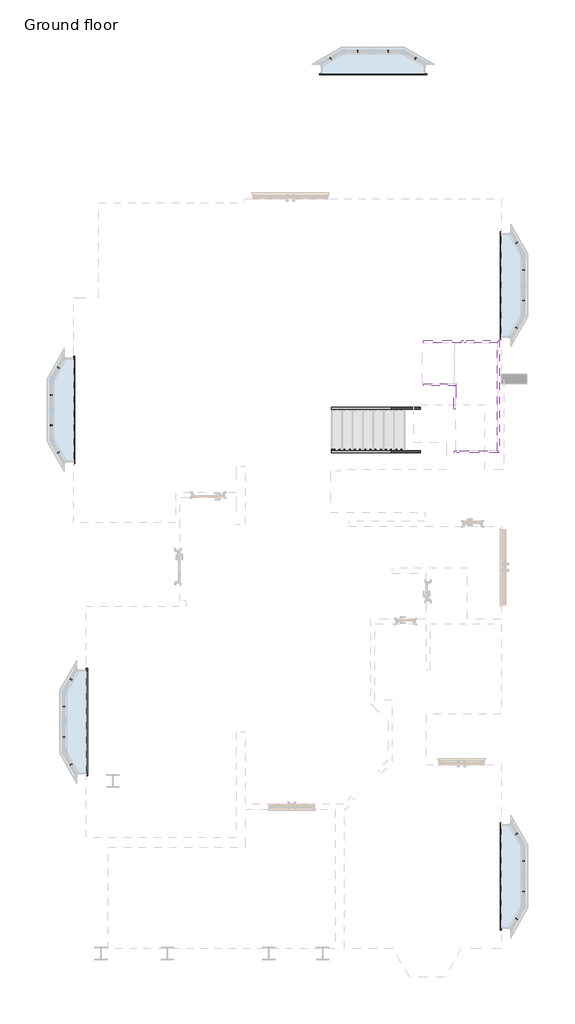
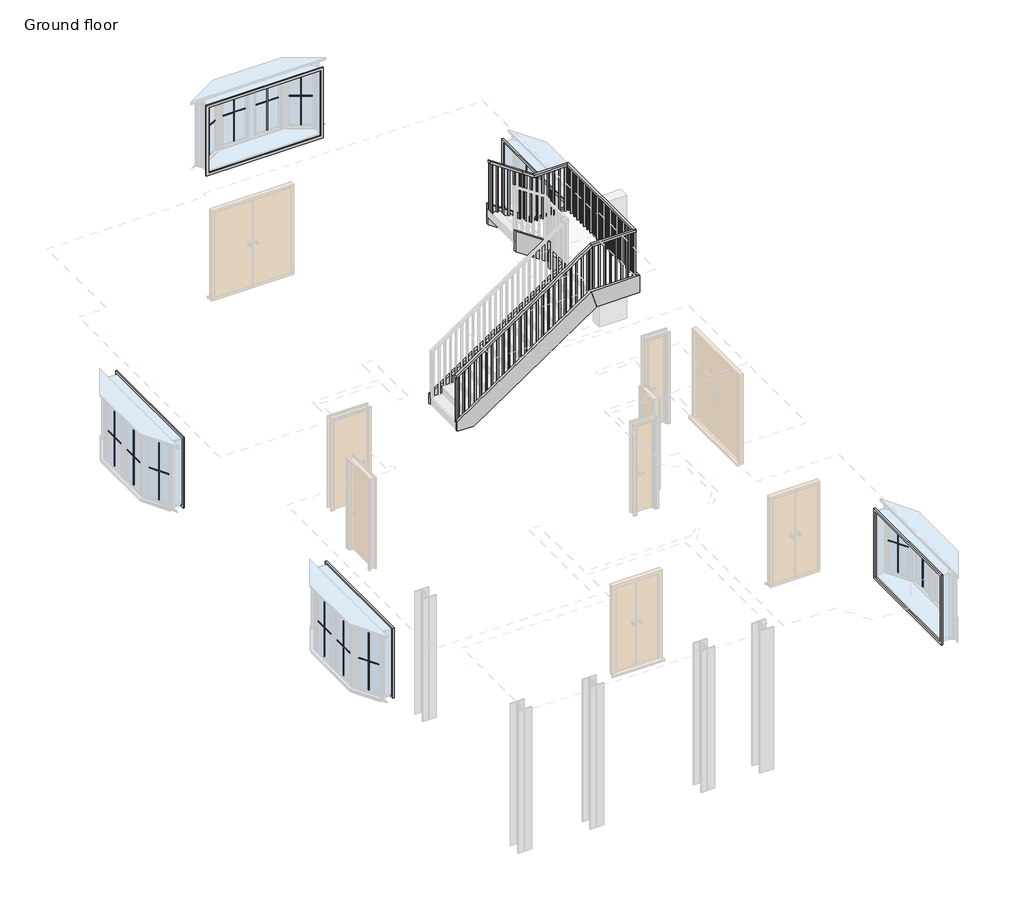
# One storey, part 2 of 2: 25 proxies, 8 members, 1 railing.
"""IFC4 building model written with IfcOpenShell, lengths in millimetres."""

import ifcopenshell
import ifcopenshell.guid

model = None  # the IFC model being written
_history = None  # IfcOwnerHistory: only IFC2X3 demands one
_inside = {}  # id of a spatial element -> (the spatial element, [elements in it])
_under = {}  # id of a project, library or spatial element -> (it, [spatial elements below it])
_declared = {}  # id of a project -> (the project, [libraries it declares])
_typed = {}  # id of a type object -> (the type object, [elements of that type])
_made_of = {}  # id of a material, layer set ... -> (it, [elements and type objects made of it])


def new_model(schema):
    """Start an empty IFC model of exactly this schema.

    Asked for "IFC4X3", IfcOpenShell would pick the latest addendum, in which some entities
    have other attributes; the version numbers below select the first issue.
    IFC2X3 requires an IfcOwnerHistory on every rooted entity: one is made here for all.
    """
    global model, _history
    if schema == "IFC4X3":
        model = ifcopenshell.file(schema_version=(4, 3, 0, 0))
    else:
        model = ifcopenshell.file(schema=schema)
    _inside.clear()
    _under.clear()
    _declared.clear()
    _typed.clear()
    _made_of.clear()
    _history = None
    if model.schema == "IFC2X3":
        org = make("IfcOrganization", Name="unknown")
        user = make(
            "IfcPersonAndOrganization",
            ThePerson=make("IfcPerson", FamilyName="unknown"),
            TheOrganization=org,
        )
        app = make(
            "IfcApplication",
            ApplicationDeveloper=org,
            Version="unknown",
            ApplicationFullName="unknown",
            ApplicationIdentifier="unknown",
        )
        _history = make(
            "IfcOwnerHistory",
            OwningUser=user,
            OwningApplication=app,
            ChangeAction="ADDED",
            CreationDate=0,
        )
    return model


def make(cls, **values):
    """One entity of the class cls with the attributes given. An attribute that is None is left unset."""
    return model.create_entity(
        cls, **{name: value for name, value in values.items() if value is not None}
    )


def rooted(cls, **values):
    """An entity with a GlobalId (a new one), such as an element, a storey or a relation."""
    return make(cls, GlobalId=ifcopenshell.guid.new(), OwnerHistory=_history, **values)


def si_unit(unit_type, name, prefix=None):
    """IfcSIUnit, for example si_unit("LENGTHUNIT", "METRE", prefix="MILLI")."""
    return make("IfcSIUnit", UnitType=unit_type, Prefix=prefix, Name=name)


def assignment(units):
    """IfcUnitAssignment: the units of a project."""
    return None if units is None else make("IfcUnitAssignment", Units=units)


def point(xyz):
    """IfcCartesianPoint."""
    return None if xyz is None else make("IfcCartesianPoint", Coordinates=xyz)


def direction(xyz):
    """IfcDirection."""
    return None if xyz is None else make("IfcDirection", DirectionRatios=xyz)


def frame(location, z_axis=None, x_axis=None):
    """IfcAxis2Placement3D, a coordinate frame: its origin and axes. An axis left out is left unset."""
    return make(
        "IfcAxis2Placement3D",
        Location=point(location),
        Axis=direction(z_axis),
        RefDirection=direction(x_axis),
    )


def origin():
    """The frame at (0, 0, 0) with its axes left unset."""
    return frame((0.0, 0.0, 0.0))


def origin_with_axes():
    """The frame at (0, 0, 0) with the z axis (0, 0, 1) and the x axis (1, 0, 0) written out."""
    return frame((0.0, 0.0, 0.0), z_axis=(0.0, 0.0, 1.0), x_axis=(1.0, 0.0, 0.0))


def place(relative_to, where):
    """IfcLocalPlacement: puts the frame where relative to a parent placement (None: the world)."""
    return make(
        "IfcLocalPlacement", PlacementRelTo=relative_to, RelativePlacement=where
    )


def context(
    kind, dimensions, precision=None, world=None, true_north=None, identifier=None
):
    """IfcGeometricRepresentationContext, for example the 3D "Model" context."""
    return make(
        "IfcGeometricRepresentationContext",
        ContextIdentifier=identifier,
        ContextType=kind,
        CoordinateSpaceDimension=dimensions,
        Precision=precision,
        WorldCoordinateSystem=world,
        TrueNorth=true_north,
    )


def project(units=None, contexts=None):
    """IfcProject with its units and contexts."""
    return rooted(
        "IfcProject",
        Name="project",
        RepresentationContexts=contexts,
        UnitsInContext=assignment(units),
    )


def spatial(cls, under=None, at=None, **own):
    """A site, building, storey or space (cls), placed at a placement, below another one or the project."""
    s = rooted(cls, ObjectPlacement=at, **own)
    if under is not None:
        _under.setdefault(under.id(), (under, []))[1].append(s)
    return s


def polyline(points):
    """IfcPolyline through the points."""
    return make("IfcPolyline", Points=[point(p) for p in points])


def outline(outer, holes=None, kind="AREA"):
    """IfcArbitraryClosedProfileDef: a profile drawn as a closed curve; with holes, ...WithVoids."""
    if holes is None:
        return make("IfcArbitraryClosedProfileDef", ProfileType=kind, OuterCurve=outer)
    return make(
        "IfcArbitraryProfileDefWithVoids",
        ProfileType=kind,
        OuterCurve=outer,
        InnerCurves=holes,
    )


def extrude(swept, where, along, depth):
    """IfcExtrudedAreaSolid: the profile swept, set in the frame where, extruded along a direction by depth."""
    return make(
        "IfcExtrudedAreaSolid",
        SweptArea=swept,
        Position=where,
        ExtrudedDirection=direction(along),
        Depth=depth,
    )


def faces_of(points, faces, orient=None, outer=None):
    """IfcFace entities. A face is a list of loops; a loop is a list of indices into points, from 0.

    orient and outer hold one flag for each loop. By default every Orientation is true, the
    first loop of a face is its IfcFaceOuterBound and the others are IfcFaceBound.
    """
    made = []
    for i, loops in enumerate(faces):
        bounds = []
        for j, loop in enumerate(loops):
            is_outer = j == 0 if outer is None else outer[i][j]
            bounds.append(
                make(
                    "IfcFaceOuterBound" if is_outer else "IfcFaceBound",
                    Bound=make("IfcPolyLoop", Polygon=[points[k] for k in loop]),
                    Orientation=True if orient is None else orient[i][j],
                )
            )
        made.append(make("IfcFace", Bounds=bounds))
    return made


def faceted_brep(points, faces, orient=None, outer=None, voids=None):
    """IfcFacetedBrep: a solid bounded by flat faces; with voids (closed shells), ...WithVoids."""
    shared = [point(p) for p in points]
    hull = make("IfcClosedShell", CfsFaces=faces_of(shared, faces, orient, outer))
    if voids is None:
        return make("IfcFacetedBrep", Outer=hull)
    return make(
        "IfcFacetedBrepWithVoids",
        Outer=hull,
        Voids=[
            make(cls, CfsFaces=faces_of(shared, fs, o, b)) for cls, fs, o, b in voids
        ],
    )


def shape(context_of_items, identifier, shape_type, items):
    """IfcShapeRepresentation: the items that make up one representation, for example the "Body"."""
    return make(
        "IfcShapeRepresentation",
        ContextOfItems=context_of_items,
        RepresentationIdentifier=identifier,
        RepresentationType=shape_type,
        Items=items,
    )


def source(mapping_origin, context_of_items, identifier, shape_type, items):
    """IfcRepresentationMap: a shape defined once, which mapped items show again and again."""
    return make(
        "IfcRepresentationMap",
        MappingOrigin=mapping_origin,
        MappedRepresentation=shape(context_of_items, identifier, shape_type, items),
    )


def transform(
    local_origin,
    x_axis=None,
    y_axis=None,
    z_axis=None,
    scale=None,
    scale2=None,
    scale3=None,
    uniform=True,
):
    """IfcCartesianTransformationOperator3D, or its non-uniform kind. x_axis, y_axis, z_axis: its Axis1, 2, 3."""
    if uniform:
        return make(
            "IfcCartesianTransformationOperator3D",
            Axis1=direction(x_axis),
            Axis2=direction(y_axis),
            LocalOrigin=point(local_origin),
            Scale=scale,
            Axis3=direction(z_axis),
        )
    return make(
        "IfcCartesianTransformationOperator3DnonUniform",
        Axis1=direction(x_axis),
        Axis2=direction(y_axis),
        LocalOrigin=point(local_origin),
        Scale=scale,
        Axis3=direction(z_axis),
        Scale2=scale2,
        Scale3=scale3,
    )


def mapped(mapping_source, mapping_target):
    """IfcMappedItem: shows the shape of a source again, moved by a transform."""
    return make(
        "IfcMappedItem", MappingSource=mapping_source, MappingTarget=mapping_target
    )


def made_of(thing, what):
    """Note that an element or type object is made of a material, layer set ...; save() writes the relation."""
    if what is not None:
        _made_of.setdefault(what.id(), (what, []))[1].append(thing)
    return thing


def element(
    cls,
    number,
    at=None,
    inside=None,
    cuts=None,
    type_object=None,
    material=None,
    context=None,
    identifier="Body",
    shape_type=None,
    held_by="IfcProductDefinitionShape",
    body=None,
    shapes=None,
    **own,
):
    """One element of the class cls, such as IfcWall. Its Tag is "e" and its number.

    at: its placement. inside: the storey or other place that contains it. cuts: it is an
    opening in that element (IfcRelVoidsElement). A single representation is given by context,
    identifier, shape_type and body (its items); several are given by shapes. held_by: the class
    of the entity that holds the representations. save() writes the other relations.
    """
    e = rooted(cls, Tag="e%d" % number, ObjectPlacement=at, **own)
    if body is not None:
        shapes = [shape(context, identifier, shape_type, body)]
    if shapes is not None:
        e.Representation = make(held_by, Representations=shapes)
    if inside is not None:
        _inside.setdefault(inside.id(), (inside, []))[1].append(e)
    if cuts is not None:
        rooted(
            "IfcRelVoidsElement", RelatingBuildingElement=cuts, RelatedOpeningElement=e
        )
    if type_object is not None:
        _typed.setdefault(type_object.id(), (type_object, []))[1].append(e)
    return made_of(e, material)


def aggregate(whole, parts):
    """IfcRelAggregates: a whole, such as a stair, and the parts it consists of."""
    return rooted("IfcRelAggregates", RelatingObject=whole, RelatedObjects=parts)


def save(model, path):
    """Write the relations noted so far, then the file.

    IfcRelAggregates (storeys below a building ...), IfcRelContainedInSpatialStructure (elements
    in a storey), IfcRelDefinesByType, IfcRelAssociatesMaterial and IfcRelDeclares: one each for
    every whole, place, type object, material and project.
    """
    for whole, parts in _under.values():
        aggregate(whole, parts)
    for where, things in _inside.values():
        rooted(
            "IfcRelContainedInSpatialStructure",
            RelatedElements=things,
            RelatingStructure=where,
        )
    for kind, things in _typed.values():
        rooted("IfcRelDefinesByType", RelatedObjects=things, RelatingType=kind)
    for what, things in _made_of.values():
        rooted("IfcRelAssociatesMaterial", RelatedObjects=things, RelatingMaterial=what)
    for by, libraries in _declared.values():
        rooted("IfcRelDeclares", RelatingContext=by, RelatedDefinitions=libraries)
    model.write(path)


def m_muntin_pattern_2x2_m_muntin_pattern_2x2_0b9f2fee(model_context):
    return source(origin(), model_context, "Body", "SweptSolid", [
        extrude(outline(polyline([(686.5, -6.35), (686.5, -246.1999152), (673.8, -246.1999152), (673.8, -6.35), (0.0, -6.35), (0.0, 6.35), (673.8, 6.35), (673.8, 246.1999152), (686.5, 246.1999152), (686.5, 6.35), (1360.3, 6.35), (1360.3, -6.35), (686.5, -6.35)])), frame((0.0, 9.525, 0.0), z_axis=(0.0, 1.0, 0.0), x_axis=(0.0, 0.0, 1.0)), (0.0, 0.0, 1.0), 12.7),
        extrude(outline(polyline([(686.5, -6.35), (686.5, -246.1999152), (673.8, -246.1999152), (673.8, -6.35), (0.0, -6.35), (0.0, 6.35), (673.8, 6.35), (673.8, 246.1999152), (686.5, 246.1999152), (686.5, 6.35), (1360.3, 6.35), (1360.3, -6.35), (686.5, -6.35)])), frame((0.0, -22.225, 0.0), z_axis=(0.0, 1.0, 0.0), x_axis=(0.0, 0.0, 1.0)), (0.0, 0.0, 1.0), 12.7),
    ])


def m_muntin_pattern_2x2_m_muntin_pattern_2x2_98e5798c(model_context):
    return source(origin(), model_context, "Body", "SweptSolid", [
        extrude(outline(polyline([(686.5, -6.35), (686.5, -223.0), (673.8, -223.0), (673.8, -6.35), (0.0, -6.35), (0.0, 6.35), (673.8, 6.35), (673.8, 223.0), (686.5, 223.0), (686.5, 6.35), (1360.3, 6.35), (1360.3, -6.35), (686.5, -6.35)])), frame((0.0, 9.525, 0.0), z_axis=(0.0, 1.0, 0.0), x_axis=(0.0, 0.0, 1.0)), (0.0, 0.0, 1.0), 12.7),
        extrude(outline(polyline([(686.5, -6.35), (686.5, -223.0), (673.8, -223.0), (673.8, -6.35), (0.0, -6.35), (0.0, 6.35), (673.8, 6.35), (673.8, 223.0), (686.5, 223.0), (686.5, 6.35), (1360.3, 6.35), (1360.3, -6.35), (686.5, -6.35)])), frame((0.0, -22.225, 0.0), z_axis=(0.0, 1.0, 0.0), x_axis=(0.0, 0.0, 1.0)), (0.0, 0.0, 1.0), 12.7),
    ])


def m_muntin_pattern_2x2_m_muntin_pattern_2x2_86194ec4(model_context):
    return source(origin(), model_context, "Body", "SweptSolid", [
        extrude(outline(polyline([(686.5, -6.35), (686.5, -223.0), (673.8, -223.0), (673.8, -6.35), (0.0, -6.35), (0.0, 6.35), (673.8, 6.35), (673.8, 223.0), (686.5, 223.0), (686.5, 6.35), (1360.3, 6.35), (1360.3, -6.35), (686.5, -6.35)])), frame((0.0, -22.225, 0.0), z_axis=(0.0, 1.0, 0.0), x_axis=(0.0, 0.0, 1.0)), (0.0, 0.0, 1.0), 12.7),
        extrude(outline(polyline([(686.5, -6.35), (686.5, -223.0), (673.8, -223.0), (673.8, -6.35), (0.0, -6.35), (0.0, 6.35), (673.8, 6.35), (673.8, 223.0), (686.5, 223.0), (686.5, 6.35), (1360.3, 6.35), (1360.3, -6.35), (686.5, -6.35)])), frame((0.0, 9.525, 0.0), z_axis=(0.0, 1.0, 0.0), x_axis=(0.0, 0.0, 1.0)), (0.0, 0.0, 1.0), 12.7),
    ])


def m_trim_window_interior_flat_picture_frame_cdca9661(model_context):
    return source(origin(), model_context, "Body", "SweptSolid", [
        extrude(outline(polyline([(1297.3, 47.3), (1297.3, -1598.1), (-1297.3, -1598.1), (-1297.3, 47.3), (1297.3, 47.3)]), holes=[polyline([(1237.3, -12.7), (-1237.3, -12.7), (-1237.3, -1538.1), (1237.3, -1538.1), (1237.3, -12.7)])]), origin_with_axes(), (0.0, 0.0, 1.0), 30.0),
    ])


model = new_model("IFC4")

# Units and contexts
model_context = context("Model", 3, world=origin())
ifc_project = project(units=[si_unit("LENGTHUNIT", "METRE", prefix="MILLI")], contexts=[model_context])

# Site, building, storey
site = spatial("IfcSite", under=ifc_project)
building = spatial("IfcBuilding", under=site)
storey = spatial("IfcBuildingStorey", under=building, Name="Ground floor", Elevation=450.0)

# Proxies
placement = place(None, origin())
m_muntin_pattern_2x2_m_muntin_pattern_2x2_shape = m_muntin_pattern_2x2_m_muntin_pattern_2x2_0b9f2fee(model_context)
element("IfcBuildingElementProxy", 1, Name="M_Muntin Pattern_2x2 : M_Muntin Pattern_2x2", ObjectType="M_Muntin Pattern_2x2 : M_Muntin Pattern_2x2", at=placement, inside=storey, context=model_context, shape_type="MappedRepresentation", body=[
    mapped(m_muntin_pattern_2x2_m_muntin_pattern_2x2_shape, transform((-7333.5440924, 632.1140304, 1170.65), x_axis=(0.0, 1.0, 0.0), y_axis=(-1.0, 0.0, 0.0), z_axis=(0.0, 0.0, 1.0))),
])
element("IfcBuildingElementProxy", 2, Name="M_Muntin Pattern_2x2 : M_Muntin Pattern_2x2", ObjectType="M_Muntin Pattern_2x2 : M_Muntin Pattern_2x2", at=placement, inside=storey, context=model_context, shape_type="MappedRepresentation", body=[
    mapped(m_muntin_pattern_2x2_m_muntin_pattern_2x2_shape, transform((-7333.5440924, 1365.8138609, 1170.65), x_axis=(0.0, 1.0, 0.0), y_axis=(-1.0, 0.0, 0.0), z_axis=(0.0, 0.0, 1.0))),
])
element("IfcBuildingElementProxy", 3, Name="M_Muntin Pattern_2x2 : M_Muntin Pattern_2x2", ObjectType="M_Muntin Pattern_2x2 : M_Muntin Pattern_2x2", at=placement, inside=storey, context=model_context, shape_type="MappedRepresentation", body=[
    mapped(m_muntin_pattern_2x2_m_muntin_pattern_2x2_shape, transform((-7028.7440924, -6902.6609696, 1170.65), x_axis=(0.0, 1.0, 0.0), y_axis=(-1.0, 0.0, 0.0), z_axis=(0.0, 0.0, 1.0))),
])
element("IfcBuildingElementProxy", 4, Name="M_Muntin Pattern_2x2 : M_Muntin Pattern_2x2", ObjectType="M_Muntin Pattern_2x2 : M_Muntin Pattern_2x2", at=placement, inside=storey, context=model_context, shape_type="MappedRepresentation", body=[
    mapped(m_muntin_pattern_2x2_m_muntin_pattern_2x2_shape, transform((-7028.7440924, -6168.9611391, 1170.65), x_axis=(0.0, 1.0, 0.0), y_axis=(-1.0, 0.0, 0.0), z_axis=(0.0, 0.0, 1.0))),
])
element("IfcBuildingElementProxy", 5, Name="M_Muntin Pattern_2x2 : M_Muntin Pattern_2x2", ObjectType="M_Muntin Pattern_2x2 : M_Muntin Pattern_2x2", at=placement, inside=storey, context=model_context, shape_type="MappedRepresentation", body=[
    mapped(m_muntin_pattern_2x2_m_muntin_pattern_2x2_shape, transform((78.5809923, 9664.9889456, 1170.65), x_axis=(1.0, 0.0, 0.0), y_axis=(0.0, 1.0, 0.0), z_axis=(0.0, 0.0, 1.0))),
])
element("IfcBuildingElementProxy", 6, Name="M_Muntin Pattern_2x2 : M_Muntin Pattern_2x2", ObjectType="M_Muntin Pattern_2x2 : M_Muntin Pattern_2x2", at=placement, inside=storey, context=model_context, shape_type="MappedRepresentation", body=[
    mapped(m_muntin_pattern_2x2_m_muntin_pattern_2x2_shape, transform((812.2808228, 9664.9889456, 1170.65), x_axis=(1.0, 0.0, 0.0), y_axis=(0.0, 1.0, 0.0), z_axis=(0.0, 0.0, 1.0))),
])
element("IfcBuildingElementProxy", 7, Name="M_Muntin Pattern_2x2 : M_Muntin Pattern_2x2", ObjectType="M_Muntin Pattern_2x2 : M_Muntin Pattern_2x2", at=placement, inside=storey, context=model_context, shape_type="MappedRepresentation", body=[
    mapped(m_muntin_pattern_2x2_m_muntin_pattern_2x2_shape, transform((4086.6559076, 4380.1138609, 1170.65), x_axis=(0.0, -1.0, 0.0), y_axis=(1.0, 0.0, 0.0), z_axis=(0.0, 0.0, 1.0))),
])
element("IfcBuildingElementProxy", 8, Name="M_Muntin Pattern_2x2 : M_Muntin Pattern_2x2", ObjectType="M_Muntin Pattern_2x2 : M_Muntin Pattern_2x2", at=placement, inside=storey, context=model_context, shape_type="MappedRepresentation", body=[
    mapped(m_muntin_pattern_2x2_m_muntin_pattern_2x2_shape, transform((4086.6559076, 3646.4140304, 1170.65), x_axis=(0.0, -1.0, 0.0), y_axis=(1.0, 0.0, 0.0), z_axis=(0.0, 0.0, 1.0))),
])
element("IfcBuildingElementProxy", 9, Name="M_Muntin Pattern_2x2 : M_Muntin Pattern_2x2", ObjectType="M_Muntin Pattern_2x2 : M_Muntin Pattern_2x2", at=placement, inside=storey, context=model_context, shape_type="MappedRepresentation", body=[
    mapped(m_muntin_pattern_2x2_m_muntin_pattern_2x2_shape, transform((4086.6559076, -9900.9861391, 1170.65), x_axis=(0.0, -1.0, 0.0), y_axis=(1.0, 0.0, 0.0), z_axis=(0.0, 0.0, 1.0))),
])
element("IfcBuildingElementProxy", 10, Name="M_Muntin Pattern_2x2 : M_Muntin Pattern_2x2", ObjectType="M_Muntin Pattern_2x2 : M_Muntin Pattern_2x2", at=placement, inside=storey, context=model_context, shape_type="MappedRepresentation", body=[
    mapped(m_muntin_pattern_2x2_m_muntin_pattern_2x2_shape, transform((4086.6559076, -10634.6859696, 1170.65), x_axis=(0.0, -1.0, 0.0), y_axis=(1.0, 0.0, 0.0), z_axis=(0.0, 0.0, 1.0))),
])
m_muntin_pattern_2x2_m_muntin_pattern_2x2_2_shape = m_muntin_pattern_2x2_m_muntin_pattern_2x2_98e5798c(model_context)
element("IfcBuildingElementProxy", 11, Name="M_Muntin Pattern_2x2 : M_Muntin Pattern_2x2", ObjectType="M_Muntin Pattern_2x2 : M_Muntin Pattern_2x2", at=placement, inside=storey, context=model_context, shape_type="MappedRepresentation", body=[
    mapped(m_muntin_pattern_2x2_m_muntin_pattern_2x2_2_shape, transform((-7162.9952004, -27.5830149, 1170.65), x_axis=(-0.4999999999999925, 0.866025403784443, 0.0), y_axis=(-0.866025403784443, -0.4999999999999925, 0.0), z_axis=(0.0, 0.0, 1.0))),
])
element("IfcBuildingElementProxy", 12, Name="M_Muntin Pattern_2x2 : M_Muntin Pattern_2x2", ObjectType="M_Muntin Pattern_2x2 : M_Muntin Pattern_2x2", at=placement, inside=storey, context=model_context, shape_type="MappedRepresentation", body=[
    mapped(m_muntin_pattern_2x2_m_muntin_pattern_2x2_2_shape, transform((-6858.1952004, -7562.3580149, 1170.65), x_axis=(-0.49999999999999245, 0.866025403784443, 0.0), y_axis=(-0.866025403784443, -0.49999999999999245, 0.0), z_axis=(0.0, 0.0, 1.0))),
])
element("IfcBuildingElementProxy", 13, Name="M_Muntin Pattern_2x2 : M_Muntin Pattern_2x2", ObjectType="M_Muntin Pattern_2x2 : M_Muntin Pattern_2x2", at=placement, inside=storey, context=model_context, shape_type="MappedRepresentation", body=[
    mapped(m_muntin_pattern_2x2_m_muntin_pattern_2x2_2_shape, transform((-581.1160529, 9494.4400536, 1170.65), x_axis=(0.8660254037844438, 0.49999999999999106, 0.0), y_axis=(-0.49999999999999106, 0.8660254037844438, 0.0), z_axis=(0.0, 0.0, 1.0))),
])
element("IfcBuildingElementProxy", 14, Name="M_Muntin Pattern_2x2 : M_Muntin Pattern_2x2", ObjectType="M_Muntin Pattern_2x2 : M_Muntin Pattern_2x2", at=placement, inside=storey, context=model_context, shape_type="MappedRepresentation", body=[
    mapped(m_muntin_pattern_2x2_m_muntin_pattern_2x2_2_shape, transform((3916.1070156, 5039.8109061, 1170.65), x_axis=(0.49999999999999245, -0.866025403784443, 0.0), y_axis=(0.866025403784443, 0.49999999999999245, 0.0), z_axis=(0.0, 0.0, 1.0))),
])
element("IfcBuildingElementProxy", 15, Name="M_Muntin Pattern_2x2 : M_Muntin Pattern_2x2", ObjectType="M_Muntin Pattern_2x2 : M_Muntin Pattern_2x2", at=placement, inside=storey, context=model_context, shape_type="MappedRepresentation", body=[
    mapped(m_muntin_pattern_2x2_m_muntin_pattern_2x2_2_shape, transform((3916.1070156, -9241.2890939, 1170.65), x_axis=(0.4999999999999924, -0.866025403784443, 0.0), y_axis=(0.866025403784443, 0.4999999999999924, 0.0), z_axis=(0.0, 0.0, 1.0))),
])
m_muntin_pattern_2x2_m_muntin_pattern_2x2_3_shape = m_muntin_pattern_2x2_m_muntin_pattern_2x2_86194ec4(model_context)
element("IfcBuildingElementProxy", 16, Name="M_Muntin Pattern_2x2 : M_Muntin Pattern_2x2", ObjectType="M_Muntin Pattern_2x2 : M_Muntin Pattern_2x2", at=placement, inside=storey, context=model_context, shape_type="MappedRepresentation", body=[
    mapped(m_muntin_pattern_2x2_m_muntin_pattern_2x2_3_shape, transform((-7162.9952004, 2025.5109061, 1170.65), x_axis=(-0.49999999999999517, -0.8660254037844415, 0.0), y_axis=(0.8660254037844415, -0.49999999999999517, 0.0), z_axis=(0.0, 0.0, 1.0))),
])
element("IfcBuildingElementProxy", 17, Name="M_Muntin Pattern_2x2 : M_Muntin Pattern_2x2", ObjectType="M_Muntin Pattern_2x2 : M_Muntin Pattern_2x2", at=placement, inside=storey, context=model_context, shape_type="MappedRepresentation", body=[
    mapped(m_muntin_pattern_2x2_m_muntin_pattern_2x2_3_shape, transform((-6858.1952004, -5509.2640939, 1170.65), x_axis=(-0.4999999999999952, -0.8660254037844415, 0.0), y_axis=(0.8660254037844415, -0.4999999999999952, 0.0), z_axis=(0.0, 0.0, 1.0))),
])
element("IfcBuildingElementProxy", 18, Name="M_Muntin Pattern_2x2 : M_Muntin Pattern_2x2", ObjectType="M_Muntin Pattern_2x2 : M_Muntin Pattern_2x2", at=placement, inside=storey, context=model_context, shape_type="MappedRepresentation", body=[
    mapped(m_muntin_pattern_2x2_m_muntin_pattern_2x2_3_shape, transform((1471.9778681, 9494.4400536, 1170.65), x_axis=(-0.8660254037844407, 0.4999999999999966, 0.0), y_axis=(-0.4999999999999966, -0.8660254037844407, 0.0), z_axis=(0.0, 0.0, 1.0))),
])
element("IfcBuildingElementProxy", 19, Name="M_Muntin Pattern_2x2 : M_Muntin Pattern_2x2", ObjectType="M_Muntin Pattern_2x2 : M_Muntin Pattern_2x2", at=placement, inside=storey, context=model_context, shape_type="MappedRepresentation", body=[
    mapped(m_muntin_pattern_2x2_m_muntin_pattern_2x2_3_shape, transform((3916.1070156, 2986.7169851, 1170.65), x_axis=(0.4999999999999952, 0.8660254037844415, 0.0), y_axis=(-0.8660254037844415, 0.4999999999999952, 0.0), z_axis=(0.0, 0.0, 1.0))),
])
element("IfcBuildingElementProxy", 20, Name="M_Muntin Pattern_2x2 : M_Muntin Pattern_2x2", ObjectType="M_Muntin Pattern_2x2 : M_Muntin Pattern_2x2", at=placement, inside=storey, context=model_context, shape_type="MappedRepresentation", body=[
    mapped(m_muntin_pattern_2x2_m_muntin_pattern_2x2_3_shape, transform((3916.1070156, -11294.3830149, 1170.65), x_axis=(0.4999999999999953, 0.8660254037844415, 0.0), y_axis=(-0.8660254037844415, 0.4999999999999953, 0.0), z_axis=(0.0, 0.0, 1.0))),
])
m_trim_window_interior_flat_picture_frame_shape = m_trim_window_interior_flat_picture_frame_cdca9661(model_context)
element("IfcBuildingElementProxy", 21, Name="M_Trim-Window-Interior-Flat : Picture Frame", ObjectType="M_Trim-Window-Interior-Flat : Picture Frame", at=placement, inside=storey, context=model_context, shape_type="MappedRepresentation", body=[
    mapped(m_trim_window_interior_flat_picture_frame_shape, transform((-6794.8190924, 998.9639456, 2600.8), x_axis=(0.0, 1.0, 0.0), y_axis=(0.0, 0.0, 1.0), z_axis=(1.0, 0.0, 0.0))),
])
element("IfcBuildingElementProxy", 22, Name="M_Trim-Window-Interior-Flat : Picture Frame", ObjectType="M_Trim-Window-Interior-Flat : Picture Frame", at=placement, inside=storey, context=model_context, shape_type="MappedRepresentation", body=[
    mapped(m_trim_window_interior_flat_picture_frame_shape, transform((-6490.0190924, -6535.8110544, 2600.8), x_axis=(0.0, 1.0, 0.0), y_axis=(0.0, 0.0, 1.0), z_axis=(1.0, 0.0, 0.0))),
])
element("IfcBuildingElementProxy", 23, Name="M_Trim-Window-Interior-Flat : Picture Frame", ObjectType="M_Trim-Window-Interior-Flat : Picture Frame", at=placement, inside=storey, context=model_context, shape_type="MappedRepresentation", body=[
    mapped(m_trim_window_interior_flat_picture_frame_shape, transform((445.4309076, 9126.2639456, 2600.8), x_axis=(1.0, 0.0, 0.0), y_axis=(0.0, 0.0, 1.0), z_axis=(0.0, -1.0, 0.0))),
])
element("IfcBuildingElementProxy", 24, Name="M_Trim-Window-Interior-Flat : Picture Frame", ObjectType="M_Trim-Window-Interior-Flat : Picture Frame", at=placement, inside=storey, context=model_context, shape_type="MappedRepresentation", body=[
    mapped(m_trim_window_interior_flat_picture_frame_shape, transform((3547.9309076, 4013.2639456, 2600.8), x_axis=(0.0, -1.0, 0.0), y_axis=(0.0, 0.0, 1.0), z_axis=(-1.0, 0.0, 0.0))),
])
element("IfcBuildingElementProxy", 25, Name="M_Trim-Window-Interior-Flat : Picture Frame", ObjectType="M_Trim-Window-Interior-Flat : Picture Frame", at=placement, inside=storey, context=model_context, shape_type="MappedRepresentation", body=[
    mapped(m_trim_window_interior_flat_picture_frame_shape, transform((3547.9309076, -10267.8360544, 2600.8), x_axis=(0.0, -1.0, 0.0), y_axis=(0.0, 0.0, 1.0), z_axis=(-1.0, 0.0, 0.0))),
])

# Members
element("IfcMember", 26, ObjectType="Stringer-50mm_Width", at=placement, inside=storey, context=model_context, shape_type="SweptSolid", body=[
    extrude(outline(polyline([(684.2596208, -554.509652), (450.0, -554.509652), (450.0, -187.0347657), (2198.4606499, 2395.490348), (2681.5137384, 2395.490348), (684.2596208, -554.509652)])), frame((0.0, 1019.7308056, 0.0), z_axis=(0.0, 1.0, 0.0), x_axis=(0.0, 0.0, 1.0)), (0.0, 0.0, 1.0), 50.0),
])
element("IfcMember", 27, ObjectType="Stringer-50mm_Width", at=placement, inside=storey, context=model_context, shape_type="SweptSolid", body=[
    extrude(outline(polyline([(684.2596208, -554.509652), (450.0, -554.509652), (450.0, -187.0347657), (2292.801214, 2534.8339907), (2692.801214, 2412.162264), (684.2596208, -554.509652)])), frame((0.0, -30.2691944, 0.0), z_axis=(0.0, 1.0, 0.0), x_axis=(0.0, 0.0, 1.0)), (0.0, 0.0, 1.0), 50.0),
])
element("IfcMember", 28, ObjectType="Stringer-50mm_Width", at=placement, inside=storey, context=model_context, shape_type="SweptSolid", body=[
    extrude(outline(polyline([(2382.2418805, 2445.490348), (2865.294969, 2445.490348), (3392.4007972, 1666.940348), (2909.3477087, 1666.940348), (2382.2418805, 2445.490348)])), frame((0.0, 1581.1308056, 0.0), z_axis=(0.0, 1.0, 0.0), x_axis=(0.0, 0.0, 1.0)), (0.0, 0.0, 1.0), 50.0),
])
element("IfcMember", 29, ObjectType="Stringer-50mm_Width", at=placement, inside=storey, context=model_context, shape_type="SweptSolid", body=[
    extrude(outline(polyline([(2292.801214, 2577.5967052), (2692.801214, 2700.2684319), (3392.4007972, 1666.940348), (2909.3477087, 1666.940348), (2292.801214, 2577.5967052)])), frame((0.0, 2631.1308056, 0.0), z_axis=(0.0, 1.0, 0.0), x_axis=(0.0, 0.0, 1.0)), (0.0, 0.0, 1.0), 50.0),
])
element("IfcMember", 30, ObjectType="Stringer-50mm_Width", at=placement, inside=storey, context=model_context, shape_type="SweptSolid", body=[
    extrude(outline(polyline([(2395.490348, 1581.1308056), (2445.490348, 1581.1308056), (2445.490348, 1019.7308056), (2395.490348, 1019.7308056), (2395.490348, 1581.1308056)])), frame((0.0, 0.0, 2292.801214), z_axis=(0.0, 0.0, 1.0), x_axis=(1.0, 0.0, 0.0)), (0.0, 0.0, 1.0), 400.0),
])
element("IfcMember", 31, ObjectType="Stringer-50mm_Width", at=placement, inside=storey, context=model_context, shape_type="Brep", body=[
    faceted_brep([(2412.162264, 19.7308056, 2692.801214), (2412.162264, -30.2691944, 2692.801214), (3495.490348, -30.2691944, 2692.801214), (3445.490348, 19.7308056, 2692.801214), (2534.8339907, 19.7308056, 2292.801214), (3445.490348, 19.7308056, 2292.801214), (2534.8339907, -30.2691944, 2292.801214), (3495.490348, -30.2691944, 2292.801214)], [[[0, 1, 2, 3]], [[4, 0, 3, 5]], [[6, 4, 5, 7]], [[1, 6, 7, 2]], [[1, 0, 4, 6]], [[2, 7, 5, 3]]]),
])
element("IfcMember", 32, ObjectType="Stringer-50mm_Width", at=placement, inside=storey, context=model_context, shape_type="SweptSolid", body=[
    extrude(outline(polyline([(3495.490348, -30.2691944), (3445.490348, 19.7308056), (3445.490348, 2631.1308056), (3495.490348, 2681.1308056), (3495.490348, -30.2691944)])), frame((0.0, 0.0, 2292.801214), z_axis=(0.0, 0.0, 1.0), x_axis=(1.0, 0.0, 0.0)), (0.0, 0.0, 1.0), 400.0),
])
element("IfcMember", 33, ObjectType="Stringer-50mm_Width", at=placement, inside=storey, context=model_context, shape_type="Brep", body=[
    faceted_brep([(3445.490348, 2631.1308056, 2692.801214), (3495.490348, 2681.1308056, 2692.801214), (2700.2684319, 2681.1308056, 2692.801214), (2700.2684319, 2631.1308056, 2692.801214), (3445.490348, 2631.1308056, 2292.801214), (2577.5967052, 2631.1308056, 2292.801214), (3495.490348, 2681.1308056, 2292.801214), (2577.5967052, 2681.1308056, 2292.801214)], [[[0, 1, 2, 3]], [[4, 0, 3, 5]], [[6, 4, 5, 7]], [[1, 6, 7, 2]], [[1, 0, 4, 6]], [[2, 7, 5, 3]]]),
])

# Railing
element("IfcRailing", 34, ObjectType="1100mm", at=placement, inside=storey, context=model_context, shape_type="SolidModel", body=[
    faceted_brep([(-554.509652, 70.1308056, 1719.2588235), (-554.509652, 70.1308056, 1658.8771875), (-554.509652, 20.1308056, 1658.8771875), (-554.509652, 20.1308056, 1719.2588235), (2445.490348, 70.1308056, 3750.3647059), (2460.8243138, 70.1308056, 3700.3647059), (2460.8243138, 20.1308056, 3700.3647059), (2445.490348, 20.1308056, 3750.3647059), (3395.090348, 70.1308056, 3750.3647059), (3395.090348, 70.1308056, 3700.3647059), (3445.090348, 20.1308056, 3700.3647059), (3445.090348, 20.1308056, 3750.3647059), (3395.090348, 2580.7308056, 3750.3647059), (3395.090348, 2580.7308056, 3700.3647059), (3445.090348, 2630.7308056, 3700.3647059), (3445.090348, 2630.7308056, 3750.3647059), (2666.940348, 2580.7308056, 3750.3647059), (2651.6063821, 2580.7308056, 3700.3647059), (2651.6063821, 2630.7308056, 3700.3647059), (2666.940348, 2630.7308056, 3750.3647059), (2416.940348, 2580.7308056, 3919.6235294), (2388.9088413, 2580.7308056, 3878.2202127), (2388.9088413, 2630.7308056, 3878.2202127), (2416.940348, 2630.7308056, 3919.6235294), (1666.940348, 2580.7308056, 4427.4), (1666.940348, 2630.7308056, 4427.4), (1666.940348, 2630.7308056, 4367.0183639), (1666.940348, 2580.7308056, 4367.0183639)], [[[0, 1, 2, 3]], [[1, 0, 4, 5]], [[2, 1, 5, 6]], [[3, 2, 6, 7]], [[0, 3, 7, 4]], [[5, 4, 8, 9]], [[6, 5, 9, 10]], [[7, 6, 10, 11]], [[4, 7, 11, 8]], [[9, 8, 12, 13]], [[10, 9, 13, 14]], [[11, 10, 14, 15]], [[8, 11, 15, 12]], [[13, 12, 16, 17]], [[14, 13, 17, 18]], [[15, 14, 18, 19]], [[12, 15, 19, 16]], [[17, 16, 20, 21]], [[18, 17, 21, 22]], [[19, 18, 22, 23]], [[16, 19, 23, 20]], [[24, 25, 26, 27]], [[21, 20, 24, 27]], [[22, 21, 27, 26]], [[23, 22, 26, 25]], [[20, 23, 25, 24]]]),
    extrude(outline(polyline([(3158.1411765, 1741.940348), (4316.2407169, 1741.940348), (4333.1665992, 1716.940348), (3158.1411765, 1716.940348), (3158.1411765, 1741.940348)])), frame((0.0, 2593.2308056, 0.0), z_axis=(0.0, 1.0, 0.0), x_axis=(0.0, 0.0, 1.0)), (0.0, 0.0, 1.0), 25.0),
    extrude(outline(polyline([(3158.1411765, 1866.940348), (4231.6113051, 1866.940348), (4248.5371875, 1841.940348), (3158.1411765, 1841.940348), (3158.1411765, 1866.940348)])), frame((0.0, 2593.2308056, 0.0), z_axis=(0.0, 1.0, 0.0), x_axis=(0.0, 0.0, 1.0)), (0.0, 0.0, 1.0), 25.0),
    extrude(outline(polyline([(2988.8823529, 1991.940348), (4146.9818933, 1991.940348), (4163.9077757, 1966.940348), (2988.8823529, 1966.940348), (2988.8823529, 1991.940348)])), frame((0.0, 2593.2308056, 0.0), z_axis=(0.0, 1.0, 0.0), x_axis=(0.0, 0.0, 1.0)), (0.0, 0.0, 1.0), 25.0),
    extrude(outline(polyline([(2988.8823529, 2116.940348), (4062.3524816, 2116.940348), (4079.2783639, 2091.940348), (2988.8823529, 2091.940348), (2988.8823529, 2116.940348)])), frame((0.0, 2593.2308056, 0.0), z_axis=(0.0, 1.0, 0.0), x_axis=(0.0, 0.0, 1.0)), (0.0, 0.0, 1.0), 25.0),
    extrude(outline(polyline([(2819.6235294, 2241.940348), (3977.7230698, 2241.940348), (3994.6489522, 2216.940348), (2819.6235294, 2216.940348), (2819.6235294, 2241.940348)])), frame((0.0, 2593.2308056, 0.0), z_axis=(0.0, 1.0, 0.0), x_axis=(0.0, 0.0, 1.0)), (0.0, 0.0, 1.0), 25.0),
    extrude(outline(polyline([(2819.6235294, 2366.940348), (3893.0936581, 2366.940348), (3910.0195404, 2341.940348), (2819.6235294, 2341.940348), (2819.6235294, 2366.940348)])), frame((0.0, 2593.2308056, 0.0), z_axis=(0.0, 1.0, 0.0), x_axis=(0.0, 0.0, 1.0)), (0.0, 0.0, 1.0), 25.0),
    extrude(outline(polyline([(2650.3647059, 2495.090348), (3806.3315851, 2495.090348), (3823.2574675, 2470.090348), (2650.3647059, 2470.090348), (2650.3647059, 2495.090348)])), frame((0.0, 2593.2308056, 0.0), z_axis=(0.0, 1.0, 0.0), x_axis=(0.0, 0.0, 1.0)), (0.0, 0.0, 1.0), 25.0),
    extrude(outline(polyline([(2650.3647059, 2620.090348), (3721.7021733, 2620.090348), (3738.6280557, 2595.090348), (2650.3647059, 2595.090348), (2650.3647059, 2620.090348)])), frame((0.0, 2593.2308056, 0.0), z_axis=(0.0, 1.0, 0.0), x_axis=(0.0, 0.0, 1.0)), (0.0, 0.0, 1.0), 25.0),
    extrude(outline(polyline([(2745.090348, 2618.2308056), (2745.090348, 2593.2308056), (2720.090348, 2593.2308056), (2720.090348, 2618.2308056), (2745.090348, 2618.2308056)])), frame((0.0, 0.0, 2650.3647059), z_axis=(0.0, 0.0, 1.0), x_axis=(1.0, 0.0, 0.0)), (0.0, 0.0, 1.0), 1050.0),
    extrude(outline(polyline([(2870.090348, 2618.2308056), (2870.090348, 2593.2308056), (2845.090348, 2593.2308056), (2845.090348, 2618.2308056), (2870.090348, 2618.2308056)])), frame((0.0, 0.0, 2650.3647059), z_axis=(0.0, 0.0, 1.0), x_axis=(1.0, 0.0, 0.0)), (0.0, 0.0, 1.0), 1050.0),
    extrude(outline(polyline([(2995.090348, 2618.2308056), (2995.090348, 2593.2308056), (2970.090348, 2593.2308056), (2970.090348, 2618.2308056), (2995.090348, 2618.2308056)])), frame((0.0, 0.0, 2650.3647059), z_axis=(0.0, 0.0, 1.0), x_axis=(1.0, 0.0, 0.0)), (0.0, 0.0, 1.0), 1050.0),
    extrude(outline(polyline([(3120.090348, 2618.2308056), (3120.090348, 2593.2308056), (3095.090348, 2593.2308056), (3095.090348, 2618.2308056), (3120.090348, 2618.2308056)])), frame((0.0, 0.0, 2650.3647059), z_axis=(0.0, 0.0, 1.0), x_axis=(1.0, 0.0, 0.0)), (0.0, 0.0, 1.0), 1050.0),
    extrude(outline(polyline([(3245.090348, 2618.2308056), (3245.090348, 2593.2308056), (3220.090348, 2593.2308056), (3220.090348, 2618.2308056), (3245.090348, 2618.2308056)])), frame((0.0, 0.0, 2650.3647059), z_axis=(0.0, 0.0, 1.0), x_axis=(1.0, 0.0, 0.0)), (0.0, 0.0, 1.0), 1050.0),
    extrude(outline(polyline([(3370.090348, 2618.2308056), (3370.090348, 2593.2308056), (3345.090348, 2593.2308056), (3345.090348, 2618.2308056), (3370.090348, 2618.2308056)])), frame((0.0, 0.0, 2650.3647059), z_axis=(0.0, 0.0, 1.0), x_axis=(1.0, 0.0, 0.0)), (0.0, 0.0, 1.0), 1050.0),
    extrude(outline(polyline([(3432.590348, 2470.1308056), (3407.590348, 2470.1308056), (3407.590348, 2495.1308056), (3432.590348, 2495.1308056), (3432.590348, 2470.1308056)])), frame((0.0, 0.0, 2650.3647059), z_axis=(0.0, 0.0, 1.0), x_axis=(1.0, 0.0, 0.0)), (0.0, 0.0, 1.0), 1050.0),
    extrude(outline(polyline([(3432.590348, 2345.1308056), (3407.590348, 2345.1308056), (3407.590348, 2370.1308056), (3432.590348, 2370.1308056), (3432.590348, 2345.1308056)])), frame((0.0, 0.0, 2650.3647059), z_axis=(0.0, 0.0, 1.0), x_axis=(1.0, 0.0, 0.0)), (0.0, 0.0, 1.0), 1050.0),
    extrude(outline(polyline([(3432.590348, 2220.1308056), (3407.590348, 2220.1308056), (3407.590348, 2245.1308056), (3432.590348, 2245.1308056), (3432.590348, 2220.1308056)])), frame((0.0, 0.0, 2650.3647059), z_axis=(0.0, 0.0, 1.0), x_axis=(1.0, 0.0, 0.0)), (0.0, 0.0, 1.0), 1050.0),
    extrude(outline(polyline([(3432.590348, 2095.1308056), (3407.590348, 2095.1308056), (3407.590348, 2120.1308056), (3432.590348, 2120.1308056), (3432.590348, 2095.1308056)])), frame((0.0, 0.0, 2650.3647059), z_axis=(0.0, 0.0, 1.0), x_axis=(1.0, 0.0, 0.0)), (0.0, 0.0, 1.0), 1050.0),
    extrude(outline(polyline([(3432.590348, 1970.1308056), (3407.590348, 1970.1308056), (3407.590348, 1995.1308056), (3432.590348, 1995.1308056), (3432.590348, 1970.1308056)])), frame((0.0, 0.0, 2650.3647059), z_axis=(0.0, 0.0, 1.0), x_axis=(1.0, 0.0, 0.0)), (0.0, 0.0, 1.0), 1050.0),
    extrude(outline(polyline([(3432.590348, 1845.1308056), (3407.590348, 1845.1308056), (3407.590348, 1870.1308056), (3432.590348, 1870.1308056), (3432.590348, 1845.1308056)])), frame((0.0, 0.0, 2650.3647059), z_axis=(0.0, 0.0, 1.0), x_axis=(1.0, 0.0, 0.0)), (0.0, 0.0, 1.0), 1050.0),
    extrude(outline(polyline([(3432.590348, 1720.1308056), (3407.590348, 1720.1308056), (3407.590348, 1745.1308056), (3432.590348, 1745.1308056), (3432.590348, 1720.1308056)])), frame((0.0, 0.0, 2650.3647059), z_axis=(0.0, 0.0, 1.0), x_axis=(1.0, 0.0, 0.0)), (0.0, 0.0, 1.0), 1050.0),
    extrude(outline(polyline([(3432.590348, 1595.1308056), (3407.590348, 1595.1308056), (3407.590348, 1620.1308056), (3432.590348, 1620.1308056), (3432.590348, 1595.1308056)])), frame((0.0, 0.0, 2650.3647059), z_axis=(0.0, 0.0, 1.0), x_axis=(1.0, 0.0, 0.0)), (0.0, 0.0, 1.0), 1050.0),
    extrude(outline(polyline([(3432.590348, 1470.1308056), (3407.590348, 1470.1308056), (3407.590348, 1495.1308056), (3432.590348, 1495.1308056), (3432.590348, 1470.1308056)])), frame((0.0, 0.0, 2650.3647059), z_axis=(0.0, 0.0, 1.0), x_axis=(1.0, 0.0, 0.0)), (0.0, 0.0, 1.0), 1050.0),
    extrude(outline(polyline([(3432.590348, 1345.1308056), (3407.590348, 1345.1308056), (3407.590348, 1370.1308056), (3432.590348, 1370.1308056), (3432.590348, 1345.1308056)])), frame((0.0, 0.0, 2650.3647059), z_axis=(0.0, 0.0, 1.0), x_axis=(1.0, 0.0, 0.0)), (0.0, 0.0, 1.0), 1050.0),
    extrude(outline(polyline([(3432.590348, 1220.1308056), (3407.590348, 1220.1308056), (3407.590348, 1245.1308056), (3432.590348, 1245.1308056), (3432.590348, 1220.1308056)])), frame((0.0, 0.0, 2650.3647059), z_axis=(0.0, 0.0, 1.0), x_axis=(1.0, 0.0, 0.0)), (0.0, 0.0, 1.0), 1050.0),
    extrude(outline(polyline([(3432.590348, 1095.1308056), (3407.590348, 1095.1308056), (3407.590348, 1120.1308056), (3432.590348, 1120.1308056), (3432.590348, 1095.1308056)])), frame((0.0, 0.0, 2650.3647059), z_axis=(0.0, 0.0, 1.0), x_axis=(1.0, 0.0, 0.0)), (0.0, 0.0, 1.0), 1050.0),
    extrude(outline(polyline([(3432.590348, 970.1308056), (3407.590348, 970.1308056), (3407.590348, 995.1308056), (3432.590348, 995.1308056), (3432.590348, 970.1308056)])), frame((0.0, 0.0, 2650.3647059), z_axis=(0.0, 0.0, 1.0), x_axis=(1.0, 0.0, 0.0)), (0.0, 0.0, 1.0), 1050.0),
    extrude(outline(polyline([(3432.590348, 845.1308056), (3407.590348, 845.1308056), (3407.590348, 870.1308056), (3432.590348, 870.1308056), (3432.590348, 845.1308056)])), frame((0.0, 0.0, 2650.3647059), z_axis=(0.0, 0.0, 1.0), x_axis=(1.0, 0.0, 0.0)), (0.0, 0.0, 1.0), 1050.0),
    extrude(outline(polyline([(3432.590348, 720.1308056), (3407.590348, 720.1308056), (3407.590348, 745.1308056), (3432.590348, 745.1308056), (3432.590348, 720.1308056)])), frame((0.0, 0.0, 2650.3647059), z_axis=(0.0, 0.0, 1.0), x_axis=(1.0, 0.0, 0.0)), (0.0, 0.0, 1.0), 1050.0),
    extrude(outline(polyline([(3432.590348, 595.1308056), (3407.590348, 595.1308056), (3407.590348, 620.1308056), (3432.590348, 620.1308056), (3432.590348, 595.1308056)])), frame((0.0, 0.0, 2650.3647059), z_axis=(0.0, 0.0, 1.0), x_axis=(1.0, 0.0, 0.0)), (0.0, 0.0, 1.0), 1050.0),
    extrude(outline(polyline([(3432.590348, 470.1308056), (3407.590348, 470.1308056), (3407.590348, 495.1308056), (3432.590348, 495.1308056), (3432.590348, 470.1308056)])), frame((0.0, 0.0, 2650.3647059), z_axis=(0.0, 0.0, 1.0), x_axis=(1.0, 0.0, 0.0)), (0.0, 0.0, 1.0), 1050.0),
    extrude(outline(polyline([(3432.590348, 345.1308056), (3407.590348, 345.1308056), (3407.590348, 370.1308056), (3432.590348, 370.1308056), (3432.590348, 345.1308056)])), frame((0.0, 0.0, 2650.3647059), z_axis=(0.0, 0.0, 1.0), x_axis=(1.0, 0.0, 0.0)), (0.0, 0.0, 1.0), 1050.0),
    extrude(outline(polyline([(3432.590348, 220.1308056), (3407.590348, 220.1308056), (3407.590348, 245.1308056), (3432.590348, 245.1308056), (3432.590348, 220.1308056)])), frame((0.0, 0.0, 2650.3647059), z_axis=(0.0, 0.0, 1.0), x_axis=(1.0, 0.0, 0.0)), (0.0, 0.0, 1.0), 1050.0),
    extrude(outline(polyline([(3432.590348, 95.1308056), (3407.590348, 95.1308056), (3407.590348, 120.1308056), (3432.590348, 120.1308056), (3432.590348, 95.1308056)])), frame((0.0, 0.0, 2650.3647059), z_axis=(0.0, 0.0, 1.0), x_axis=(1.0, 0.0, 0.0)), (0.0, 0.0, 1.0), 1050.0),
    extrude(outline(polyline([(3370.490348, 32.6308056), (3370.490348, 57.6308056), (3395.490348, 57.6308056), (3395.490348, 32.6308056), (3370.490348, 32.6308056)])), frame((0.0, 0.0, 2650.3647059), z_axis=(0.0, 0.0, 1.0), x_axis=(1.0, 0.0, 0.0)), (0.0, 0.0, 1.0), 1050.0),
    extrude(outline(polyline([(3245.490348, 32.6308056), (3245.490348, 57.6308056), (3270.490348, 57.6308056), (3270.490348, 32.6308056), (3245.490348, 32.6308056)])), frame((0.0, 0.0, 2650.3647059), z_axis=(0.0, 0.0, 1.0), x_axis=(1.0, 0.0, 0.0)), (0.0, 0.0, 1.0), 1050.0),
    extrude(outline(polyline([(3120.490348, 32.6308056), (3120.490348, 57.6308056), (3145.490348, 57.6308056), (3145.490348, 32.6308056), (3120.490348, 32.6308056)])), frame((0.0, 0.0, 2650.3647059), z_axis=(0.0, 0.0, 1.0), x_axis=(1.0, 0.0, 0.0)), (0.0, 0.0, 1.0), 1050.0),
    extrude(outline(polyline([(2995.490348, 32.6308056), (2995.490348, 57.6308056), (3020.490348, 57.6308056), (3020.490348, 32.6308056), (2995.490348, 32.6308056)])), frame((0.0, 0.0, 2650.3647059), z_axis=(0.0, 0.0, 1.0), x_axis=(1.0, 0.0, 0.0)), (0.0, 0.0, 1.0), 1050.0),
    extrude(outline(polyline([(2870.490348, 32.6308056), (2870.490348, 57.6308056), (2895.490348, 57.6308056), (2895.490348, 32.6308056), (2870.490348, 32.6308056)])), frame((0.0, 0.0, 2650.3647059), z_axis=(0.0, 0.0, 1.0), x_axis=(1.0, 0.0, 0.0)), (0.0, 0.0, 1.0), 1050.0),
    extrude(outline(polyline([(2745.490348, 32.6308056), (2745.490348, 57.6308056), (2770.490348, 57.6308056), (2770.490348, 32.6308056), (2745.490348, 32.6308056)])), frame((0.0, 0.0, 2650.3647059), z_axis=(0.0, 0.0, 1.0), x_axis=(1.0, 0.0, 0.0)), (0.0, 0.0, 1.0), 1050.0),
    extrude(outline(polyline([(2620.490348, 32.6308056), (2620.490348, 57.6308056), (2645.490348, 57.6308056), (2645.490348, 32.6308056), (2620.490348, 32.6308056)])), frame((0.0, 0.0, 2650.3647059), z_axis=(0.0, 0.0, 1.0), x_axis=(1.0, 0.0, 0.0)), (0.0, 0.0, 1.0), 1050.0),
    extrude(outline(polyline([(2495.490348, 32.6308056), (2495.490348, 57.6308056), (2520.490348, 57.6308056), (2520.490348, 32.6308056), (2495.490348, 32.6308056)])), frame((0.0, 0.0, 2650.3647059), z_axis=(0.0, 0.0, 1.0), x_axis=(1.0, 0.0, 0.0)), (0.0, 0.0, 1.0), 1050.0),
    extrude(outline(polyline([(3639.2054228, 2370.490348), (2481.1058824, 2370.490348), (2481.1058824, 2395.490348), (3656.1313051, 2395.490348), (3639.2054228, 2370.490348)])), frame((0.0, 32.6308056, 0.0), z_axis=(0.0, 1.0, 0.0), x_axis=(0.0, 0.0, 1.0)), (0.0, 0.0, 1.0), 25.0),
    extrude(outline(polyline([(3554.576011, 2245.490348), (2481.1058824, 2245.490348), (2481.1058824, 2270.490348), (3571.5018933, 2270.490348), (3554.576011, 2245.490348)])), frame((0.0, 32.6308056, 0.0), z_axis=(0.0, 1.0, 0.0), x_axis=(0.0, 0.0, 1.0)), (0.0, 0.0, 1.0), 25.0),
    extrude(outline(polyline([(3469.9465992, 2120.490348), (2311.8470588, 2120.490348), (2311.8470588, 2145.490348), (3486.8724816, 2145.490348), (3469.9465992, 2120.490348)])), frame((0.0, 32.6308056, 0.0), z_axis=(0.0, 1.0, 0.0), x_axis=(0.0, 0.0, 1.0)), (0.0, 0.0, 1.0), 25.0),
    extrude(outline(polyline([(3385.3171875, 1995.490348), (2311.8470588, 1995.490348), (2311.8470588, 2020.490348), (3402.2430698, 2020.490348), (3385.3171875, 1995.490348)])), frame((0.0, 32.6308056, 0.0), z_axis=(0.0, 1.0, 0.0), x_axis=(0.0, 0.0, 1.0)), (0.0, 0.0, 1.0), 25.0),
    extrude(outline(polyline([(3300.6877757, 1870.490348), (2142.5882353, 1870.490348), (2142.5882353, 1895.490348), (3317.6136581, 1895.490348), (3300.6877757, 1870.490348)])), frame((0.0, 32.6308056, 0.0), z_axis=(0.0, 1.0, 0.0), x_axis=(0.0, 0.0, 1.0)), (0.0, 0.0, 1.0), 25.0),
    extrude(outline(polyline([(3216.0583639, 1745.490348), (2142.5882353, 1745.490348), (2142.5882353, 1770.490348), (3232.9842463, 1770.490348), (3216.0583639, 1745.490348)])), frame((0.0, 32.6308056, 0.0), z_axis=(0.0, 1.0, 0.0), x_axis=(0.0, 0.0, 1.0)), (0.0, 0.0, 1.0), 25.0),
    extrude(outline(polyline([(3131.4289522, 1620.490348), (1973.3294118, 1620.490348), (1973.3294118, 1645.490348), (3148.3548345, 1645.490348), (3131.4289522, 1620.490348)])), frame((0.0, 32.6308056, 0.0), z_axis=(0.0, 1.0, 0.0), x_axis=(0.0, 0.0, 1.0)), (0.0, 0.0, 1.0), 25.0),
    extrude(outline(polyline([(3046.7995404, 1495.490348), (1973.3294118, 1495.490348), (1973.3294118, 1520.490348), (3063.7254228, 1520.490348), (3046.7995404, 1495.490348)])), frame((0.0, 32.6308056, 0.0), z_axis=(0.0, 1.0, 0.0), x_axis=(0.0, 0.0, 1.0)), (0.0, 0.0, 1.0), 25.0),
    extrude(outline(polyline([(2962.1701286, 1370.490348), (1804.0705882, 1370.490348), (1804.0705882, 1395.490348), (2979.096011, 1395.490348), (2962.1701286, 1370.490348)])), frame((0.0, 32.6308056, 0.0), z_axis=(0.0, 1.0, 0.0), x_axis=(0.0, 0.0, 1.0)), (0.0, 0.0, 1.0), 25.0),
    extrude(outline(polyline([(2877.5407169, 1245.490348), (1804.0705882, 1245.490348), (1804.0705882, 1270.490348), (2894.4665992, 1270.490348), (2877.5407169, 1245.490348)])), frame((0.0, 32.6308056, 0.0), z_axis=(0.0, 1.0, 0.0), x_axis=(0.0, 0.0, 1.0)), (0.0, 0.0, 1.0), 25.0),
    extrude(outline(polyline([(2792.9113051, 1120.490348), (1634.8117647, 1120.490348), (1634.8117647, 1145.490348), (2809.8371875, 1145.490348), (2792.9113051, 1120.490348)])), frame((0.0, 32.6308056, 0.0), z_axis=(0.0, 1.0, 0.0), x_axis=(0.0, 0.0, 1.0)), (0.0, 0.0, 1.0), 25.0),
    extrude(outline(polyline([(2708.2818933, 995.490348), (1634.8117647, 995.490348), (1634.8117647, 1020.490348), (2725.2077757, 1020.490348), (2708.2818933, 995.490348)])), frame((0.0, 32.6308056, 0.0), z_axis=(0.0, 1.0, 0.0), x_axis=(0.0, 0.0, 1.0)), (0.0, 0.0, 1.0), 25.0),
    extrude(outline(polyline([(2623.6524816, 870.490348), (1465.5529412, 870.490348), (1465.5529412, 895.490348), (2640.5783639, 895.490348), (2623.6524816, 870.490348)])), frame((0.0, 32.6308056, 0.0), z_axis=(0.0, 1.0, 0.0), x_axis=(0.0, 0.0, 1.0)), (0.0, 0.0, 1.0), 25.0),
    extrude(outline(polyline([(2539.0230698, 745.490348), (1465.5529412, 745.490348), (1465.5529412, 770.490348), (2555.9489522, 770.490348), (2539.0230698, 745.490348)])), frame((0.0, 32.6308056, 0.0), z_axis=(0.0, 1.0, 0.0), x_axis=(0.0, 0.0, 1.0)), (0.0, 0.0, 1.0), 25.0),
    extrude(outline(polyline([(2454.3936581, 620.490348), (1296.2941176, 620.490348), (1296.2941176, 645.490348), (2471.3195404, 645.490348), (2454.3936581, 620.490348)])), frame((0.0, 32.6308056, 0.0), z_axis=(0.0, 1.0, 0.0), x_axis=(0.0, 0.0, 1.0)), (0.0, 0.0, 1.0), 25.0),
    extrude(outline(polyline([(2369.7642463, 495.490348), (1296.2941176, 495.490348), (1296.2941176, 520.490348), (2386.6901286, 520.490348), (2369.7642463, 495.490348)])), frame((0.0, 32.6308056, 0.0), z_axis=(0.0, 1.0, 0.0), x_axis=(0.0, 0.0, 1.0)), (0.0, 0.0, 1.0), 25.0),
    extrude(outline(polyline([(2285.1348345, 370.490348), (1127.0352941, 370.490348), (1127.0352941, 395.490348), (2302.0607169, 395.490348), (2285.1348345, 370.490348)])), frame((0.0, 32.6308056, 0.0), z_axis=(0.0, 1.0, 0.0), x_axis=(0.0, 0.0, 1.0)), (0.0, 0.0, 1.0), 25.0),
    extrude(outline(polyline([(2200.5054228, 245.490348), (1127.0352941, 245.490348), (1127.0352941, 270.490348), (2217.4313051, 270.490348), (2200.5054228, 245.490348)])), frame((0.0, 32.6308056, 0.0), z_axis=(0.0, 1.0, 0.0), x_axis=(0.0, 0.0, 1.0)), (0.0, 0.0, 1.0), 25.0),
    extrude(outline(polyline([(2115.876011, 120.490348), (957.7764706, 120.490348), (957.7764706, 145.490348), (2132.8018933, 145.490348), (2115.876011, 120.490348)])), frame((0.0, 32.6308056, 0.0), z_axis=(0.0, 1.0, 0.0), x_axis=(0.0, 0.0, 1.0)), (0.0, 0.0, 1.0), 25.0),
    extrude(outline(polyline([(2031.2465992, -4.509652), (957.7764706, -4.509652), (957.7764706, 20.490348), (2048.1724816, 20.490348), (2031.2465992, -4.509652)])), frame((0.0, 32.6308056, 0.0), z_axis=(0.0, 1.0, 0.0), x_axis=(0.0, 0.0, 1.0)), (0.0, 0.0, 1.0), 25.0),
    extrude(outline(polyline([(1946.6171875, -129.509652), (788.5176471, -129.509652), (788.5176471, -104.509652), (1963.5430698, -104.509652), (1946.6171875, -129.509652)])), frame((0.0, 32.6308056, 0.0), z_axis=(0.0, 1.0, 0.0), x_axis=(0.0, 0.0, 1.0)), (0.0, 0.0, 1.0), 25.0),
    extrude(outline(polyline([(1861.9877757, -254.509652), (788.5176471, -254.509652), (788.5176471, -229.509652), (1878.9136581, -229.509652), (1861.9877757, -254.509652)])), frame((0.0, 32.6308056, 0.0), z_axis=(0.0, 1.0, 0.0), x_axis=(0.0, 0.0, 1.0)), (0.0, 0.0, 1.0), 25.0),
    extrude(outline(polyline([(1777.3583639, -379.509652), (619.2588235, -379.509652), (619.2588235, -354.509652), (1794.2842463, -354.509652), (1777.3583639, -379.509652)])), frame((0.0, 32.6308056, 0.0), z_axis=(0.0, 1.0, 0.0), x_axis=(0.0, 0.0, 1.0)), (0.0, 0.0, 1.0), 25.0),
    extrude(outline(polyline([(1692.7289522, -504.509652), (619.2588235, -504.509652), (619.2588235, -479.509652), (1709.6548345, -479.509652), (1692.7289522, -504.509652)])), frame((0.0, 32.6308056, 0.0), z_axis=(0.0, 1.0, 0.0), x_axis=(0.0, 0.0, 1.0)), (0.0, 0.0, 1.0), 25.0),
    extrude(outline(polyline([(2650.3647059, 2429.440348), (3850.7789522, 2429.440348), (3867.7048345, 2404.440348), (2650.3647059, 2404.440348), (2650.3647059, 2429.440348)])), frame((0.0, 2593.2308056, 0.0), z_axis=(0.0, 1.0, 0.0), x_axis=(0.0, 0.0, 1.0)), (0.0, 0.0, 1.0), 25.0),
    extrude(outline(polyline([(3432.590348, 2593.2308056), (3407.590348, 2593.2308056), (3407.590348, 2618.2308056), (3432.590348, 2618.2308056), (3432.590348, 2593.2308056)])), frame((0.0, 0.0, 2650.3647059), z_axis=(0.0, 0.0, 1.0), x_axis=(1.0, 0.0, 0.0)), (0.0, 0.0, 1.0), 1050.0),
    extrude(outline(polyline([(3407.590348, 32.6308056), (3407.590348, 57.6308056), (3432.590348, 57.6308056), (3432.590348, 32.6308056), (3407.590348, 32.6308056)])), frame((0.0, 0.0, 2650.3647059), z_axis=(0.0, 0.0, 1.0), x_axis=(1.0, 0.0, 0.0)), (0.0, 0.0, 1.0), 1050.0),
    extrude(outline(polyline([(3681.5201286, 2432.990348), (2650.3647059, 2432.990348), (2650.3647059, 2457.990348), (3698.446011, 2457.990348), (3681.5201286, 2432.990348)])), frame((0.0, 32.6308056, 0.0), z_axis=(0.0, 1.0, 0.0), x_axis=(0.0, 0.0, 1.0)), (0.0, 0.0, 1.0), 25.0),
    extrude(outline(polyline([(3158.1411765, 1691.940348), (4350.0924816, 1691.940348), (4367.0183639, 1666.940348), (3158.1411765, 1666.940348), (3158.1411765, 1691.940348)])), frame((0.0, 2593.2308056, 0.0), z_axis=(0.0, 1.0, 0.0), x_axis=(0.0, 0.0, 1.0)), (0.0, 0.0, 1.0), 25.0),
    extrude(outline(polyline([(1658.8771875, -554.509652), (619.2588235, -554.509652), (619.2588235, -529.509652), (1675.8030698, -529.509652), (1658.8771875, -554.509652)])), frame((0.0, 32.6308056, 0.0), z_axis=(0.0, 1.0, 0.0), x_axis=(0.0, 0.0, 1.0)), (0.0, 0.0, 1.0), 25.0),
])

save(model, "model.ifc")

# Revit data of these elements
# Type "M_Muntin Pattern_2x2 : M_Muntin Pattern_2x2"
#   Width [instance default] = 1200 mm
#   Thickness = 12.7 mm
#   Height [instance default] = 1200 mm
#   Distance = 19.05 mm
#   Interior Material [instance default] = none
#   Exterior Material [instance default] = none
#   Default Elevation = 0
# Type "M_Trim-Window-Interior-Flat : Picture Frame"
#   Trim Thickness_Picture Frame = 30 mm
#   Trim Width = 60 mm
#   Trim Thickness_with Sill = 20 mm
#   Sill Thickness = 30 mm
#   Opening Width [instance default] = 600 mm
#   Opening Height [instance default] = 900 mm
#   Default Elevation = 1200 mm
#   Sill = no
#   Picture Frame = yes
#   Trim Material [instance default] = none
# Type "1100mm"
#   built-in parameter 1008612 = 0.019685 (stored number, unit not read)
#   built-in parameter 1008611 = 0.019685 (stored number, unit not read)
#   built-in parameter 1008609 = 0.902231 (stored number, unit not read)
#   built-in parameter 1008604 = 0.19685 (stored number, unit not read)
#   built-in parameter 1008603 = 0.164042 (stored number, unit not read)
#   Railing Height = 1100 mm
#   built-in parameter 1008630 = 2
#   built-in parameter 1008610 = 2
#   built-in parameter 1008608 = 1
#   built-in parameter 1008618 = Baluster_Square : 25mm
# Elements 1, 2, 3, 4, 5, 6, 7, 8, 9, 10 (IfcBuildingElementProxy, "M_Muntin Pattern_2x2 : M_Muntin Pattern_2x2")
#   Width = 492.4 mm
#   Height = 1360.3 mm
#   Interior Material = Wood - Stained
#   Exterior Material = Clad - White
#   Phase Created = New Construction
#   Materials on its faces: "Clad - White", "Wood - Stained"
# Elements 11, 12, 13, 14, 15, 16, 17, 18, 19, 20 (IfcBuildingElementProxy, "M_Muntin Pattern_2x2 : M_Muntin Pattern_2x2")
#   Width = 446 mm
#   Height = 1360.3 mm
#   Interior Material = Wood - Stained
#   Exterior Material = Clad - White
#   Phase Created = New Construction
#   Materials on its faces: "Clad - White", "Wood - Stained"
# Elements 21, 22, 23, 24, 25 (IfcBuildingElementProxy, "M_Trim-Window-Interior-Flat : Picture Frame")
#   Opening Width = 2500 mm
#   Opening Height = 1550.8 mm
#   Trim Material = Wood - Stained
#   Phase Created = New Construction
#   Materials on its faces: "Wood - Stained"
# Elements 26, 27, 28, 29, 30, 31, 32, 33 (IfcMember, "Stringer-50mm_Width")
#   Phase Created = New Construction
# Element 34 (IfcRailing, "1100mm")
#   Phase Created = New Construction
# Materials
#   "Clad - White": class "Wood", colour RGB 242 242 238, transparency 0, Cost = 0
#   "Wood - Stained": class "Wood", colour RGB 227 170 128, transparency 0, Cost = 0
